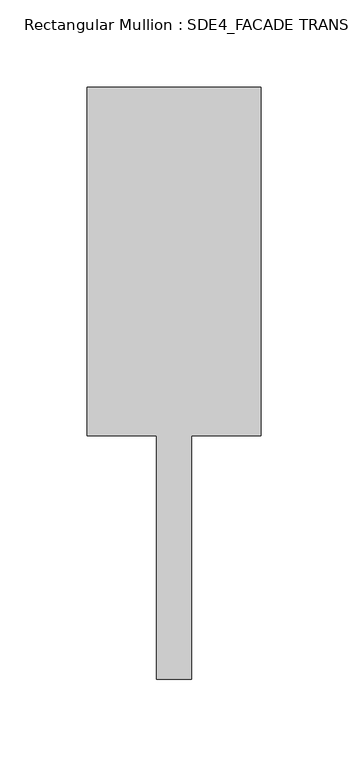
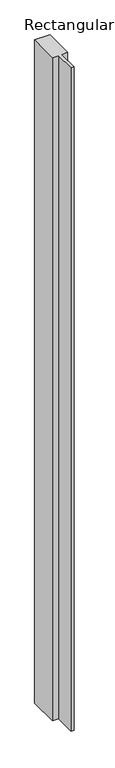
"""IFC4 building model written with IfcOpenShell, lengths in millimetres: member geometry, Rectangular Mullion : SDE4_FACADE TRANSOM TYPE 1."""

import ifcopenshell
import ifcopenshell.guid

model = None  # the IFC model being written
_history = None  # IfcOwnerHistory: only IFC2X3 demands one
_inside = {}  # id of a spatial element -> (the spatial element, [elements in it])
_under = {}  # id of a project, library or spatial element -> (it, [spatial elements below it])
_declared = {}  # id of a project -> (the project, [libraries it declares])
_typed = {}  # id of a type object -> (the type object, [elements of that type])
_made_of = {}  # id of a material, layer set ... -> (it, [elements and type objects made of it])


def new_model(schema):
    """Start an empty IFC model of exactly this schema.

    Asked for "IFC4X3", IfcOpenShell would pick the latest addendum, in which some entities
    have other attributes; the version numbers below select the first issue.
    IFC2X3 requires an IfcOwnerHistory on every rooted entity: one is made here for all.
    """
    global model, _history
    if schema == "IFC4X3":
        model = ifcopenshell.file(schema_version=(4, 3, 0, 0))
    else:
        model = ifcopenshell.file(schema=schema)
    _inside.clear()
    _under.clear()
    _declared.clear()
    _typed.clear()
    _made_of.clear()
    _history = None
    if model.schema == "IFC2X3":
        org = make("IfcOrganization", Name="unknown")
        user = make(
            "IfcPersonAndOrganization",
            ThePerson=make("IfcPerson", FamilyName="unknown"),
            TheOrganization=org,
        )
        app = make(
            "IfcApplication",
            ApplicationDeveloper=org,
            Version="unknown",
            ApplicationFullName="unknown",
            ApplicationIdentifier="unknown",
        )
        _history = make(
            "IfcOwnerHistory",
            OwningUser=user,
            OwningApplication=app,
            ChangeAction="ADDED",
            CreationDate=0,
        )
    return model


def make(cls, **values):
    """One entity of the class cls with the attributes given. An attribute that is None is left unset."""
    return model.create_entity(
        cls, **{name: value for name, value in values.items() if value is not None}
    )


def rooted(cls, **values):
    """An entity with a GlobalId (a new one), such as an element, a storey or a relation."""
    return make(cls, GlobalId=ifcopenshell.guid.new(), OwnerHistory=_history, **values)


def si_unit(unit_type, name, prefix=None):
    """IfcSIUnit, for example si_unit("LENGTHUNIT", "METRE", prefix="MILLI")."""
    return make("IfcSIUnit", UnitType=unit_type, Prefix=prefix, Name=name)


def assignment(units):
    """IfcUnitAssignment: the units of a project."""
    return None if units is None else make("IfcUnitAssignment", Units=units)


def point(xyz):
    """IfcCartesianPoint."""
    return None if xyz is None else make("IfcCartesianPoint", Coordinates=xyz)


def direction(xyz):
    """IfcDirection."""
    return None if xyz is None else make("IfcDirection", DirectionRatios=xyz)


def frame(location, z_axis=None, x_axis=None):
    """IfcAxis2Placement3D, a coordinate frame: its origin and axes. An axis left out is left unset."""
    return make(
        "IfcAxis2Placement3D",
        Location=point(location),
        Axis=direction(z_axis),
        RefDirection=direction(x_axis),
    )


def origin():
    """The frame at (0, 0, 0) with its axes left unset."""
    return frame((0.0, 0.0, 0.0))


def place(relative_to, where):
    """IfcLocalPlacement: puts the frame where relative to a parent placement (None: the world)."""
    return make(
        "IfcLocalPlacement", PlacementRelTo=relative_to, RelativePlacement=where
    )


def context(
    kind, dimensions, precision=None, world=None, true_north=None, identifier=None
):
    """IfcGeometricRepresentationContext, for example the 3D "Model" context."""
    return make(
        "IfcGeometricRepresentationContext",
        ContextIdentifier=identifier,
        ContextType=kind,
        CoordinateSpaceDimension=dimensions,
        Precision=precision,
        WorldCoordinateSystem=world,
        TrueNorth=true_north,
    )


def project(units=None, contexts=None):
    """IfcProject with its units and contexts."""
    return rooted(
        "IfcProject",
        Name="project",
        RepresentationContexts=contexts,
        UnitsInContext=assignment(units),
    )


def spatial(cls, under=None, at=None, **own):
    """A site, building, storey or space (cls), placed at a placement, below another one or the project."""
    s = rooted(cls, ObjectPlacement=at, **own)
    if under is not None:
        _under.setdefault(under.id(), (under, []))[1].append(s)
    return s


def polyline(points):
    """IfcPolyline through the points."""
    return make("IfcPolyline", Points=[point(p) for p in points])


def outline(outer, holes=None, kind="AREA"):
    """IfcArbitraryClosedProfileDef: a profile drawn as a closed curve; with holes, ...WithVoids."""
    if holes is None:
        return make("IfcArbitraryClosedProfileDef", ProfileType=kind, OuterCurve=outer)
    return make(
        "IfcArbitraryProfileDefWithVoids",
        ProfileType=kind,
        OuterCurve=outer,
        InnerCurves=holes,
    )


def extrude(swept, where, along, depth):
    """IfcExtrudedAreaSolid: the profile swept, set in the frame where, extruded along a direction by depth."""
    return make(
        "IfcExtrudedAreaSolid",
        SweptArea=swept,
        Position=where,
        ExtrudedDirection=direction(along),
        Depth=depth,
    )


def shape(context_of_items, identifier, shape_type, items):
    """IfcShapeRepresentation: the items that make up one representation, for example the "Body"."""
    return make(
        "IfcShapeRepresentation",
        ContextOfItems=context_of_items,
        RepresentationIdentifier=identifier,
        RepresentationType=shape_type,
        Items=items,
    )


def source(mapping_origin, context_of_items, identifier, shape_type, items):
    """IfcRepresentationMap: a shape defined once, which mapped items show again and again."""
    return make(
        "IfcRepresentationMap",
        MappingOrigin=mapping_origin,
        MappedRepresentation=shape(context_of_items, identifier, shape_type, items),
    )


def transform(
    local_origin,
    x_axis=None,
    y_axis=None,
    z_axis=None,
    scale=None,
    scale2=None,
    scale3=None,
    uniform=True,
):
    """IfcCartesianTransformationOperator3D, or its non-uniform kind. x_axis, y_axis, z_axis: its Axis1, 2, 3."""
    if uniform:
        return make(
            "IfcCartesianTransformationOperator3D",
            Axis1=direction(x_axis),
            Axis2=direction(y_axis),
            LocalOrigin=point(local_origin),
            Scale=scale,
            Axis3=direction(z_axis),
        )
    return make(
        "IfcCartesianTransformationOperator3DnonUniform",
        Axis1=direction(x_axis),
        Axis2=direction(y_axis),
        LocalOrigin=point(local_origin),
        Scale=scale,
        Axis3=direction(z_axis),
        Scale2=scale2,
        Scale3=scale3,
    )


def mapped(mapping_source, mapping_target):
    """IfcMappedItem: shows the shape of a source again, moved by a transform."""
    return make(
        "IfcMappedItem", MappingSource=mapping_source, MappingTarget=mapping_target
    )


def made_of(thing, what):
    """Note that an element or type object is made of a material, layer set ...; save() writes the relation."""
    if what is not None:
        _made_of.setdefault(what.id(), (what, []))[1].append(thing)
    return thing


def element(
    cls,
    number,
    at=None,
    inside=None,
    cuts=None,
    type_object=None,
    material=None,
    context=None,
    identifier="Body",
    shape_type=None,
    held_by="IfcProductDefinitionShape",
    body=None,
    shapes=None,
    **own,
):
    """One element of the class cls, such as IfcWall. Its Tag is "e" and its number.

    at: its placement. inside: the storey or other place that contains it. cuts: it is an
    opening in that element (IfcRelVoidsElement). A single representation is given by context,
    identifier, shape_type and body (its items); several are given by shapes. held_by: the class
    of the entity that holds the representations. save() writes the other relations.
    """
    e = rooted(cls, Tag="e%d" % number, ObjectPlacement=at, **own)
    if body is not None:
        shapes = [shape(context, identifier, shape_type, body)]
    if shapes is not None:
        e.Representation = make(held_by, Representations=shapes)
    if inside is not None:
        _inside.setdefault(inside.id(), (inside, []))[1].append(e)
    if cuts is not None:
        rooted(
            "IfcRelVoidsElement", RelatingBuildingElement=cuts, RelatedOpeningElement=e
        )
    if type_object is not None:
        _typed.setdefault(type_object.id(), (type_object, []))[1].append(e)
    return made_of(e, material)


def aggregate(whole, parts):
    """IfcRelAggregates: a whole, such as a stair, and the parts it consists of."""
    return rooted("IfcRelAggregates", RelatingObject=whole, RelatedObjects=parts)


def save(model, path):
    """Write the relations noted so far, then the file.

    IfcRelAggregates (storeys below a building ...), IfcRelContainedInSpatialStructure (elements
    in a storey), IfcRelDefinesByType, IfcRelAssociatesMaterial and IfcRelDeclares: one each for
    every whole, place, type object, material and project.
    """
    for whole, parts in _under.values():
        aggregate(whole, parts)
    for where, things in _inside.values():
        rooted(
            "IfcRelContainedInSpatialStructure",
            RelatedElements=things,
            RelatingStructure=where,
        )
    for kind, things in _typed.values():
        rooted("IfcRelDefinesByType", RelatedObjects=things, RelatingType=kind)
    for what, things in _made_of.values():
        rooted("IfcRelAssociatesMaterial", RelatedObjects=things, RelatingMaterial=what)
    for by, libraries in _declared.values():
        rooted("IfcRelDeclares", RelatingContext=by, RelatedDefinitions=libraries)
    model.write(path)


def rectangular_mullion_sde4_facade_transom_type_1_bfc05bd6(model_context):
    return source(origin(), model_context, "Body", "SweptSolid", [
        extrude(outline(polyline([(50.0, 132.5), (50.0, -67.5), (10.0, -67.5), (10.0, -207.5), (-10.0, -207.5), (-10.0, -67.5), (-50.0, -67.5), (-50.0, 132.5), (50.0, 132.5)])), frame((0.0, 0.0, -4578.0), z_axis=(0.0, 0.0, 1.0), x_axis=(1.0, 0.0, 0.0)), (0.0, 0.0, 1.0), 4578.0),
    ])


if __name__ == "__main__":
    model = new_model("IFC4")
    model_context = context("Model", 3, world=origin())
    ifc_project = project(units=[si_unit("LENGTHUNIT", "METRE", prefix="MILLI")], contexts=[model_context])
    site = spatial("IfcSite", under=ifc_project)
    building = spatial("IfcBuilding", under=site)
    placement = place(None, origin())
    rectangular_mullion_sde4_facade_transom_type_1_shape = rectangular_mullion_sde4_facade_transom_type_1_bfc05bd6(model_context)
    element("IfcMember", 1, ObjectType="Rectangular Mullion : SDE4_FACADE TRANSOM TYPE 1", at=placement, inside=building, context=model_context, shape_type="MappedRepresentation", body=[
        mapped(rectangular_mullion_sde4_facade_transom_type_1_shape, transform((0.0, 0.0, 0.0), x_axis=(1.0, 0.0, 0.0), y_axis=(0.0, 1.0, 0.0), z_axis=(0.0, 0.0, 1.0))),
    ])
    save(model, "model.ifc")

# Revit data of these elements
# Type "Rectangular Mullion : SDE4_FACADE TRANSOM TYPE 1"
#   built-in parameter 1007322 = 1.11549 (stored number, unit not read)
#   built-in parameter 1007321 = 0.164042 (stored number, unit not read)
#   built-in parameter 1007320 = 0.164042 (stored number, unit not read)
